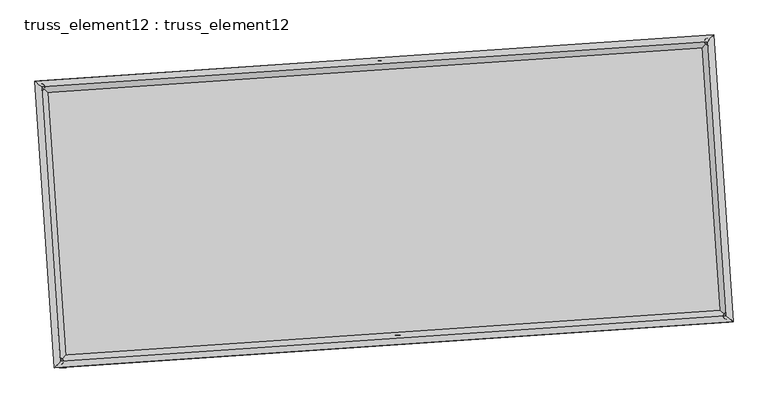
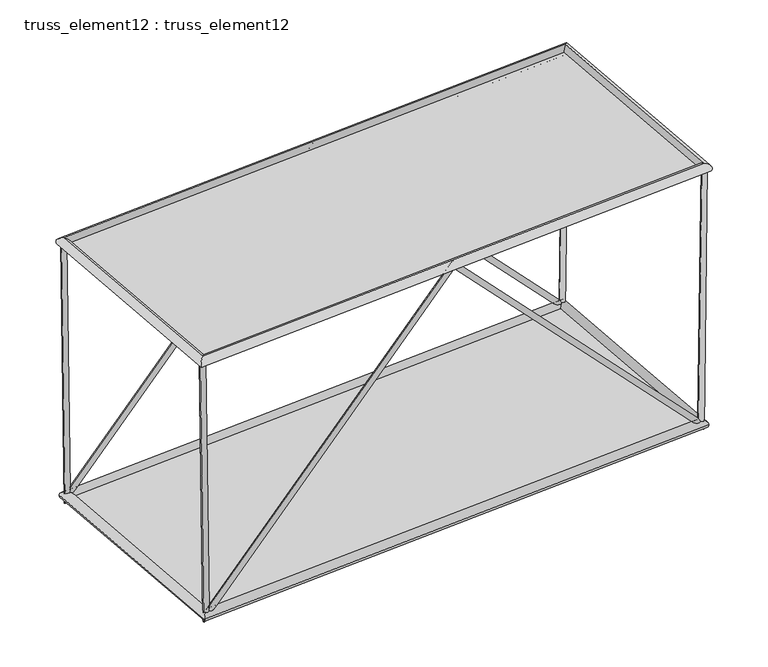
"""IFC4 building model written with IfcOpenShell, lengths in millimetres: plate geometry, truss_element12 : truss_element12."""

from ifc_helpers import new_model, si_unit, frame, origin, origin_with_axes, place, context, project, spatial, polyline, circle_curve, ellipse_curve, outline, extrude, source, transform, mapped, element, save
from ifc_brep_helpers import plane_surface, cylinder_surface, advanced_brep


def truss_element12_truss_element12_8e82c5bd(model_context):
    return source(origin(), model_context, "Body", "SolidModel", [
        advanced_brep(
        [(-3731.8869442, 2271.6592401, 5000.2192941), (-3830.9813422, 2258.2985761, 4998.880287), (-3666.5774651, 2276.1124452, 122.499402), (-3762.4094178, 2262.9742349, -122.499402), (1063.116068, 2598.6122679, 5071.6784027), (1063.5732809, 2592.0396499, 4927.4371453), (5793.9872263, 2921.1923885, 122.5077755), (5890.7737507, 2921.1881, -122.5077755), (5858.1279304, 2925.5658993, 5000.2232822), (5958.1190537, 2925.7801202, 4998.9082326)],
        [
            (0, 1, circle_curve(frame((-3781.4341432, 2264.9789081, 4999.5497906), z_axis=(-0.013388140355827645, -0.0009128863977796117, 0.9999099581143482), x_axis=(-0.13360683337915732, 0.9910340218161442, -0.0008841251678223183)), 50.0)),
            (1, 0, circle_curve(frame((-3781.4341432, 2264.9789081, 4999.5497906), z_axis=(-0.013388140355827645, -0.0009128863977796117, 0.9999099581143482), x_axis=(-0.13360683337915732, 0.9910340218161442, -0.0008841251678223183)), 50.0)),
            (0, 2),
            (2, 3, ellipse_curve(frame((-3714.4934414, 2269.54334, 0.0), z_axis=(-0.9282671693555781, -0.06329500960449433, 0.36648847738469154), x_axis=(0.36563946873946984, 0.02493156544759802, 0.9304225899795482)), 131.9466513, 50.0)),
            (3, 1),
            (3, 2, ellipse_curve(frame((-3714.4934414, 2269.54334, 0.0), z_axis=(-0.9282671693555781, -0.06329500960449433, 0.36648847738469154), x_axis=(0.36563946873946984, 0.02493156544759802, 0.9304225899795482)), 131.9466513, 50.0)),
            (2, 4),
            (4, 5, ellipse_curve(frame((1063.3446744, 2595.3259589, 4999.557774), z_axis=(-0.9976833941197891, -0.0680282380953912, -6.260394869337924e-05), x_axis=(6.245892014005556e-05, 4.258836337772687e-06, -0.9999999980403728)), 72.2776719, 50.0)),
            (5, 3),
            (5, 4, ellipse_curve(frame((1063.3446744, 2595.3259589, 4999.557774), z_axis=(-0.9976833941197891, -0.0680282380953912, -6.260394869337924e-05), x_axis=(6.245892014005556e-05, 4.258836337772687e-06, -0.9999999980403728)), 72.2776719, 50.0)),
            (4, 6),
            (6, 7, ellipse_curve(frame((5842.3804885, 2921.1902443, 0.0), z_axis=(-0.9282003652529641, -0.06329045448668236, -0.36665842457951714), x_axis=(-0.36580902223395634, -0.024943126655857368, 0.9303556307589407)), 131.9651677, 50.0)),
            (7, 5),
            (7, 6, ellipse_curve(frame((5842.3804885, 2921.1902443, 0.0), z_axis=(-0.9282003652529641, -0.06329045448668236, -0.36665842457951714), x_axis=(-0.36580902223395634, -0.024943126655857368, 0.9303556307589407)), 131.9651677, 50.0)),
            (8, 9, circle_curve(frame((5908.1234921, 2925.6730098, 4999.5657574), z_axis=(0.013148600710357648, 0.0008965530999268896, 0.9999131514746162), x_axis=(-0.002153813196862378, 0.9999973035626637, -0.0008683064638333599)), 50.0)),
            (9, 8, circle_curve(frame((5908.1234921, 2925.6730098, 4999.5657574), z_axis=(0.013148600710357648, 0.0008965530999268896, 0.9999131514746162), x_axis=(-0.002153813196862378, 0.9999973035626637, -0.0008683064638333599)), 50.0)),
            (6, 8),
            (9, 7),
        ],
        [
            plane_surface(frame((-3781.4341432, 2314.9788872, 4999.595439), z_axis=(-0.01338814035582826, -0.0009128863977758225, 0.9999099581143482), x_axis=(0.9999103748325711, -1.2222946706330628e-05, 0.013388134776246131))),
            cylinder_surface(frame((-3781.4341432, 2264.9789081, 4999.5497906), z_axis=(-0.013388140355827645, -0.0009128863977796117, 0.9999099581143482), x_axis=(-0.13360683337915732, 0.9910340218161442, -0.0008841251678223183)), 50.0),
            cylinder_surface(frame((-3714.4934414, 2269.54334, 0.0), z_axis=(-0.6901288948828247, -0.04705726591652543, -0.722154915632562), x_axis=(-0.02041150749335854, 0.9987523807925791, -0.04557468840270432)), 50.0),
            cylinder_surface(frame((1063.3446744, 2595.3259589, 4999.557774), z_axis=(-0.6902190995054749, -0.04706341662684697, 0.7220682997426625), x_axis=(-0.11534365552593137, 0.9922793184891172, -0.04558064532988163)), 50.0),
            plane_surface(frame((5908.1234921, 2875.6730298, 4999.6105889), z_axis=(0.01314860071035912, 0.0008965530999253627, 0.9999131514746162), x_axis=(0.9999135534131737, -1.1789437882825396e-05, -0.013148595424972613))),
            cylinder_surface(frame((5842.3804885, 2921.1902443, 0.0), z_axis=(-0.013148600710357651, -0.0008965530999268898, -0.9999131514746165), x_axis=(-0.002153813196862378, 0.9999973035626637, -0.0008683064638333599)), 50.0),
        ],
        [
            (0, [[1, 2]]),
            (1, [[-1, 3, 4, 5]]),
            (1, [[-2, -5, 6, -3]]),
            (2, [[-4, 7, 8, 9]]),
            (2, [[-6, -9, 10, -7]]),
            (3, [[-8, 11, 12, 13]]),
            (3, [[-10, -13, 14, -11]]),
            (4, [[15, 16]]),
            (5, [[-12, 17, -16, 18]]),
            (5, [[-14, -18, -15, -17]]),
        ],
    ),
        advanced_brep(
        [(-3459.7739913, -1719.0743442, 5000.2192941), (-3558.8683893, -1732.4350082, 4998.880287), (-3394.4645122, -1714.6211391, 122.499402), (-3490.2964649, -1727.7593494, -122.499402), (1335.2290209, -1392.1213164, 5071.6784027), (1335.6862338, -1398.6939344, 4927.4371453), (6066.1001792, -1069.5411958, 122.5077755), (6162.8867037, -1069.5454843, -122.5077755), (6130.2408833, -1065.167685, 5000.2232822), (6230.2320067, -1064.9534641, 4998.9082326)],
        [
            (0, 1, circle_curve(frame((-3509.3211903, -1725.7546762, 4999.5497906), z_axis=(-0.013388140355828339, -0.0009128863977796623, 0.9999099581143481), x_axis=(-0.13360683337915777, 0.9910340218161441, -0.0008841251678223668)), 50.0)),
            (1, 0, circle_curve(frame((-3509.3211903, -1725.7546762, 4999.5497906), z_axis=(-0.013388140355828339, -0.0009128863977796623, 0.9999099581143481), x_axis=(-0.13360683337915777, 0.9910340218161441, -0.0008841251678223668)), 50.0)),
            (0, 2),
            (2, 3, ellipse_curve(frame((-3442.3804885, -1721.1902443, 0.0), z_axis=(-0.9282671693555784, -0.06329500960449469, 0.3664884773846907), x_axis=(0.36563946873946884, 0.024931565447598097, 0.9304225899795485)), 131.9466513, 50.0)),
            (3, 1),
            (3, 2, ellipse_curve(frame((-3442.3804885, -1721.1902443, 0.0), z_axis=(-0.9282671693555784, -0.06329500960449469, 0.3664884773846907), x_axis=(0.36563946873946884, 0.024931565447598097, 0.9304225899795485)), 131.9466513, 50.0)),
            (2, 4),
            (4, 5, ellipse_curve(frame((1335.4576273, -1395.4076254, 4999.557774), z_axis=(-0.9976833941197891, -0.06802823809539131, -6.260394869402122e-05), x_axis=(6.245892014067052e-05, 4.258836337570893e-06, -0.9999999980403728)), 72.2776719, 50.0)),
            (5, 3),
            (5, 4, ellipse_curve(frame((1335.4576273, -1395.4076254, 4999.557774), z_axis=(-0.9976833941197891, -0.06802823809539131, -6.260394869402122e-05), x_axis=(6.245892014067052e-05, 4.258836337570893e-06, -0.9999999980403728)), 72.2776719, 50.0)),
            (4, 6),
            (6, 7, ellipse_curve(frame((6114.4934414, -1069.54334, 0.0), z_axis=(-0.9282003652529639, -0.06329045448668222, -0.3666584245795172), x_axis=(-0.36580902223395667, -0.02494312665585735, 0.9303556307589408)), 131.9651677, 50.0)),
            (7, 5),
            (7, 6, ellipse_curve(frame((6114.4934414, -1069.54334, 0.0), z_axis=(-0.9282003652529639, -0.06329045448668222, -0.3666584245795172), x_axis=(-0.36580902223395667, -0.02494312665585735, 0.9303556307589408)), 131.9651677, 50.0)),
            (8, 9, circle_curve(frame((6180.236445, -1065.0605745, 4999.5657574), z_axis=(0.013148600710357764, 0.0008965530999268809, 0.9999131514746162), x_axis=(-0.002153813196862232, 0.9999973035626636, -0.0008683064638333527)), 50.0)),
            (9, 8, circle_curve(frame((6180.236445, -1065.0605745, 4999.5657574), z_axis=(0.013148600710357764, 0.0008965530999268809, 0.9999131514746162), x_axis=(-0.002153813196862232, 0.9999973035626636, -0.0008683064638333527)), 50.0)),
            (6, 8),
            (9, 7),
        ],
        [
            plane_surface(frame((-3509.3211903, -1675.7546971, 4999.595439), z_axis=(-0.01338814035582826, -0.0009128863977758175, 0.9999099581143482), x_axis=(0.9999103748325711, -1.2222946706330628e-05, 0.013388134776246131))),
            cylinder_surface(frame((-3509.3211903, -1725.7546762, 4999.5497906), z_axis=(-0.013388140355828339, -0.0009128863977796623, 0.9999099581143481), x_axis=(-0.13360683337915777, 0.9910340218161441, -0.0008841251678223668)), 50.0),
            cylinder_surface(frame((-3442.3804885, -1721.1902443, 0.0), z_axis=(-0.6901288948828239, -0.04705726591652563, -0.7221549156325626), x_axis=(-0.02041150749335876, 0.9987523807925791, -0.04557468840270436)), 50.0),
            cylinder_surface(frame((1335.4576273, -1395.4076254, 4999.557774), z_axis=(-0.690219099505475, -0.047063416626846884, 0.7220682997426622), x_axis=(-0.11534365552593126, 0.9922793184891172, -0.045580645329881674)), 50.0),
            plane_surface(frame((6180.236445, -1115.0605545, 4999.6105889), z_axis=(0.01314860071035912, 0.0008965530999253614, 0.9999131514746162), x_axis=(0.9999135534131737, -1.1789437883269485e-05, -0.013148595424972613))),
            cylinder_surface(frame((6114.4934414, -1069.54334, 0.0), z_axis=(-0.013148600710357764, -0.0008965530999268809, -0.9999131514746162), x_axis=(-0.002153813196862232, 0.9999973035626636, -0.0008683064638333527)), 50.0),
        ],
        [
            (0, [[1, 2]]),
            (1, [[-1, 3, 4, 5]]),
            (1, [[-2, -5, 6, -3]]),
            (2, [[-4, 7, 8, 9]]),
            (2, [[-6, -9, 10, -7]]),
            (3, [[-8, 11, 12, 13]]),
            (3, [[-10, -13, 14, -11]]),
            (4, [[15, 16]]),
            (5, [[-12, 17, -16, 18]]),
            (5, [[-14, -18, -15, -17]]),
        ],
    ),
        advanced_brep(
        [(-3509.3170033, -1725.7500357, 4909.5497907), (-3509.3253772, -1725.7593168, 5089.5497905), (-3781.4389213, 2264.9829373, 5089.5497905), (-3781.4293651, 2264.9748788, 4909.5497907), (5908.1273838, 2925.6776302, 5089.5657573), (5908.1196003, 2925.6683893, 4909.5657575), (6180.2409278, -1065.0646239, 5089.5657573), (6180.2319621, -1065.0565252, 4909.5657575)],
        [
            (0, 1, ellipse_curve(frame((-3509.3211903, -1725.7546762, 4999.5497906), z_axis=(-0.7535719234045052, 0.6573654662781452, -1.1624966718516507e-06), x_axis=(-0.6573654662771268, -0.7535719234053935, -1.1624966718515976e-06)), 127.2792206, 90.0)),
            (1, 2),
            (2, 3, ellipse_curve(frame((-3781.4341432, 2264.9789081, 4999.5497906), z_axis=(-0.6573654662771266, -0.7535719234053936, -1.1624966705901006e-06), x_axis=(0.7535719234045052, -0.6573654662781453, 1.1624966705901538e-06)), 127.2792206, 90.0)),
            (3, 0),
            (1, 0, ellipse_curve(frame((-3509.3211903, -1725.7546762, 4999.5497906), z_axis=(-0.7535719234045052, 0.6573654662781452, -1.1624966718516507e-06), x_axis=(-0.6573654662771268, -0.7535719234053935, -1.1624966718515976e-06)), 127.2792206, 90.0)),
            (3, 2, ellipse_curve(frame((-3781.4341432, 2264.9789081, 4999.5497906), z_axis=(-0.6573654662771266, -0.7535719234053936, -1.1624966705901006e-06), x_axis=(0.7535719234045052, -0.6573654662781453, 1.1624966705901538e-06)), 127.2792206, 90.0)),
            (2, 4),
            (4, 5, ellipse_curve(frame((5908.1234921, 2925.6730098, 4999.5657574), z_axis=(-0.7535719234045045, 0.657365466278146, -1.1624966736529165e-06), x_axis=(-0.6573654662771276, -0.7535719234053929, -1.1624966675273385e-06)), 127.2792206, 90.0)),
            (5, 3),
            (5, 4, ellipse_curve(frame((5908.1234921, 2925.6730098, 4999.5657574), z_axis=(-0.7535719234045045, 0.657365466278146, -1.1624966736529165e-06), x_axis=(-0.6573654662771276, -0.7535719234053929, -1.1624966675273385e-06)), 127.2792206, 90.0)),
            (4, 6),
            (6, 7, ellipse_curve(frame((6180.236445, -1065.0605745, 4999.5657574), z_axis=(0.6573654662771274, 0.7535719234053929, 1.1624966687888353e-06), x_axis=(-0.7535719234045046, 0.657365466278146, -1.1624966749144135e-06)), 127.2792206, 90.0)),
            (7, 5),
            (7, 6, ellipse_curve(frame((6180.236445, -1065.0605745, 4999.5657574), z_axis=(0.6573654662771274, 0.7535719234053929, 1.1624966687888353e-06), x_axis=(-0.7535719234045046, 0.657365466278146, -1.1624966749144135e-06)), 127.2792206, 90.0)),
            (6, 1),
            (0, 7),
        ],
        [
            cylinder_surface(frame((-3509.3211903, -1725.7546762, 4999.5497906), z_axis=(0.06802823822870178, -0.9976833960748765, 0.0), x_axis=(-0.9976833948316877, -0.06802823814393347, -4.992144956552851e-05)), 90.0),
            cylinder_surface(frame((-3781.4341432, 2264.9789081, 4999.5497906), z_axis=(-0.9976833960735284, -0.06802823822861073, -1.644018557762127e-06), x_axis=(-0.06802823807024047, 0.9976833949176204, -4.8277431009682214e-05)), 90.0),
            cylinder_surface(frame((5908.1234921, 2925.6730098, 4999.5657574), z_axis=(-0.06802823822869981, 0.9976833960748768, 0.0), x_axis=(0.9976833949900581, 0.06802823815473016, -4.663341244950445e-05)), 90.0),
            cylinder_surface(frame((6180.236445, -1065.0605745, 4999.5657574), z_axis=(0.9976833960735283, 0.06802823822861062, 1.6440185595461528e-06), x_axis=(0.06802823822861061, -0.9976833949068217, -4.827743100280322e-05)), 90.0),
        ],
        [
            (0, [[1, 2, 3, 4]]),
            (0, [[5, -4, 6, -2]]),
            (1, [[-3, 7, 8, 9]]),
            (1, [[-6, -9, 10, -7]]),
            (2, [[-8, 11, 12, 13]]),
            (2, [[-10, -13, 14, -11]]),
            (3, [[-12, 15, -1, 16]]),
            (3, [[-14, -16, -5, -15]]),
        ],
    ),
        advanced_brep(
        [(-3358.7115243, -1625.2761972, 0.0), (-3526.0494527, -1817.1042913, 0.0), (-3810.4074885, 2353.2123043, 0.0), (-3618.5793943, 2185.8743758, 0.0), (5926.0494527, 3017.1042913, 0.0), (5758.7115243, 2825.2761972, 0.0), (6210.4074885, -1153.2123043, 0.0), (6018.5793943, -985.8743758, 0.0)],
        [
            (0, 1, ellipse_curve(frame((-3442.3804885, -1721.1902443, 0.0), z_axis=(-0.7535719234054579, 0.6573654662780808, 0.0), x_axis=(-0.6573654662780808, -0.753571923405458, 0.0)), 127.2792206, 90.0)),
            (1, 2),
            (2, 3, ellipse_curve(frame((-3714.4934414, 2269.54334, 0.0), z_axis=(-0.6573654662780806, -0.7535719234054582, 0.0), x_axis=(0.7535719234054582, -0.6573654662780805, 0.0)), 127.2792206, 90.0)),
            (3, 0),
            (1, 0, ellipse_curve(frame((-3442.3804885, -1721.1902443, 0.0), z_axis=(-0.7535719234054579, 0.6573654662780808, 0.0), x_axis=(-0.6573654662780808, -0.753571923405458, 0.0)), 127.2792206, 90.0)),
            (3, 2, ellipse_curve(frame((-3714.4934414, 2269.54334, 0.0), z_axis=(-0.6573654662780806, -0.7535719234054582, 0.0), x_axis=(0.7535719234054582, -0.6573654662780805, 0.0)), 127.2792206, 90.0)),
            (2, 4),
            (4, 5, ellipse_curve(frame((5842.3804885, 2921.1902443, 0.0), z_axis=(-0.7535719234054572, 0.6573654662780816, 0.0), x_axis=(-0.6573654662780819, -0.7535719234054571, 0.0)), 127.2792206, 90.0)),
            (5, 3),
            (5, 4, ellipse_curve(frame((5842.3804885, 2921.1902443, 0.0), z_axis=(-0.7535719234054572, 0.6573654662780816, 0.0), x_axis=(-0.6573654662780819, -0.7535719234054571, 0.0)), 127.2792206, 90.0)),
            (4, 6),
            (6, 7, ellipse_curve(frame((6114.4934414, -1069.54334, 0.0), z_axis=(0.6573654662780819, 0.7535719234054572, 0.0), x_axis=(-0.7535719234054573, 0.6573654662780816, 0.0)), 127.2792206, 90.0)),
            (7, 5),
            (7, 6, ellipse_curve(frame((6114.4934414, -1069.54334, 0.0), z_axis=(0.6573654662780819, 0.7535719234054572, 0.0), x_axis=(-0.7535719234054573, 0.6573654662780816, 0.0)), 127.2792206, 90.0)),
            (6, 1),
            (0, 7),
        ],
        [
            cylinder_surface(frame((-3442.3804885, -1721.1902443, 0.0), z_axis=(0.06802823822870138, -0.9976833960748765, 0.0), x_axis=(-0.9976833960748765, -0.06802823822870138, 0.0)), 90.0),
            cylinder_surface(frame((-3714.4934414, 2269.54334, 0.0), z_axis=(-0.9976833960748767, -0.0680282382287016, 0.0), x_axis=(-0.0680282382287016, 0.9976833960748767, 0.0)), 90.0),
            cylinder_surface(frame((5842.3804885, 2921.1902443, 0.0), z_axis=(-0.06802823822869875, 0.9976833960748769, 0.0), x_axis=(0.9976833960748769, 0.06802823822869875, 0.0)), 90.0),
            cylinder_surface(frame((6114.4934414, -1069.54334, 0.0), z_axis=(0.9976833960748767, 0.06802823822870119, 0.0), x_axis=(0.06802823822870119, -0.9976833960748767, 0.0)), 90.0),
        ],
        [
            (0, [[1, 2, 3, 4]]),
            (0, [[5, -4, 6, -2]]),
            (1, [[-3, 7, 8, 9]]),
            (1, [[-6, -9, 10, -7]]),
            (2, [[-8, 11, 12, 13]]),
            (2, [[-10, -13, 14, -11]]),
            (3, [[-12, 15, -1, 16]]),
            (3, [[-14, -16, -5, -15]]),
        ],
    ),
        extrude(outline(polyline([(-3442.3804885, -1721.1902443), (-3714.4934414, 2269.54334), (5842.3804885, 2921.1902443), (6114.4934414, -1069.54334), (-3442.3804885, -1721.1902443)])), origin_with_axes(), (0.0, 0.0, 1.0), 20.0),
        extrude(outline(polyline([(-2000.0, 4856.0283119), (2000.0, 4856.0283119), (2000.0, -4856.0283119), (-2000.0, -4856.0283119), (-2000.0, 4856.0283119)])), frame((1199.4011509, 599.9591668, 4999.557774), z_axis=(-1.6402100179182737e-06, -1.1183968609984865e-07, 0.9999999999986486), x_axis=(-0.06802823822870034, 0.9976833960748767, 0.0)), (0.0, 0.0, 1.0), 20.0),
    ])


if __name__ == "__main__":
    model = new_model("IFC4")
    model_context = context("Model", 3, world=origin())
    ifc_project = project(units=[si_unit("LENGTHUNIT", "METRE", prefix="MILLI")], contexts=[model_context])
    site = spatial("IfcSite", under=ifc_project)
    building = spatial("IfcBuilding", under=site)
    placement = place(None, origin())
    truss_element12_truss_element12_shape = truss_element12_truss_element12_8e82c5bd(model_context)
    element("IfcPlate", 1, ObjectType="truss_element12 : truss_element12", at=placement, inside=building, context=model_context, shape_type="MappedRepresentation", body=[
        mapped(truss_element12_truss_element12_shape, transform((0.0, 0.0, 0.0), x_axis=(1.0, 0.0, 0.0), y_axis=(0.0, 1.0, 0.0), z_axis=(0.0, 0.0, 1.0))),
    ])
    save(model, "model.ifc")

# Revit data of these elements
# Type "truss_element12 : truss_element12"
#   steellbar1 = 90 mm
#   steelbar2 = 50 mm
#   offset1 = 5000 mm
#   M = Default Roof
# Element 1 (IfcPlate, "truss_element12 : truss_element12")
#   Materials on its faces: "Default Roof"
# Materials
#   "Default Roof": class "Miscellaneous", colour RGB 0 127 0, transparency 0, Comments = "Rendering appearance not upgraded Rendering appearance not upgraded ", Cost = 0
